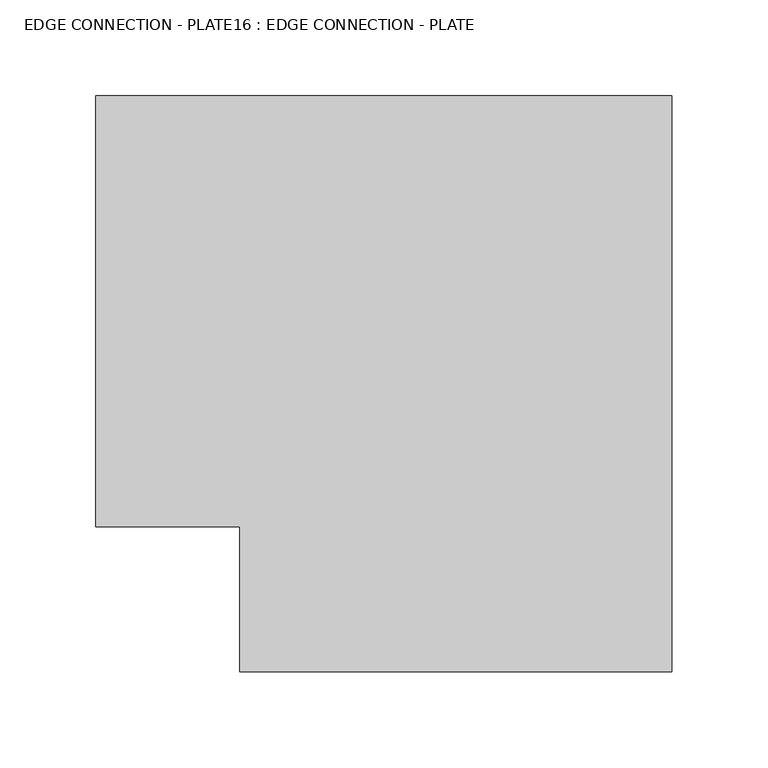
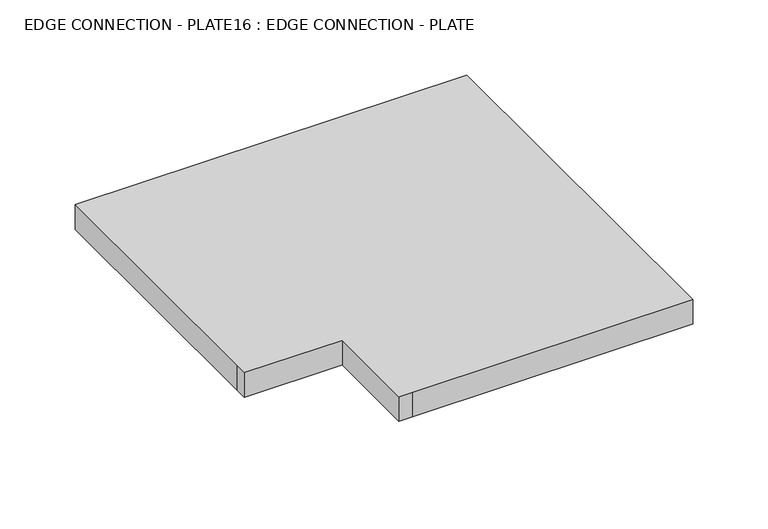
"""IFC4 building model written with IfcOpenShell, lengths in millimetres: fastener geometry, EDGE CONNECTION - PLATE16 : EDGE CONNECTION - PLATE."""

from ifc_helpers import new_model, si_unit, frame, origin, place, context, project, spatial, polyline, outline, extrude, source, transform, mapped, element, save


def edge_connection_plate16_edge_connection_plate_eba559da(model_context):
    return source(origin(), model_context, "Body", "SweptSolid", [
        extrude(outline(polyline([(5700.0, 25499.5208589), (6000.0, 25499.5208589), (6000.0, 25199.5208589), (5784.862, 25199.5208589), (5774.862, 25199.5208589), (5774.862, 25275.0508589), (5700.0, 25275.0508589), (5700.0, 25285.0508589), (5700.0, 25499.5208589)])), frame((0.0, 0.0, 200.0), z_axis=(0.0, 0.0, 1.0), x_axis=(1.0, 0.0, 0.0)), (0.0, 0.0, 1.0), 20.0),
    ])


if __name__ == "__main__":
    model = new_model("IFC4")
    model_context = context("Model", 3, world=origin())
    ifc_project = project(units=[si_unit("LENGTHUNIT", "METRE", prefix="MILLI")], contexts=[model_context])
    site = spatial("IfcSite", under=ifc_project)
    building = spatial("IfcBuilding", under=site)
    placement = place(None, origin())
    edge_connection_plate16_edge_connection_plate_shape = edge_connection_plate16_edge_connection_plate_eba559da(model_context)
    element("IfcFastener", 1, ObjectType="EDGE CONNECTION - PLATE16 : EDGE CONNECTION - PLATE", at=placement, inside=building, context=model_context, shape_type="MappedRepresentation", body=[
        mapped(edge_connection_plate16_edge_connection_plate_shape, transform((0.0, 0.0, 0.0), x_axis=(1.0, 0.0, 0.0), y_axis=(0.0, 1.0, 0.0), z_axis=(0.0, 0.0, 1.0))),
    ])
    save(model, "model.ifc")
